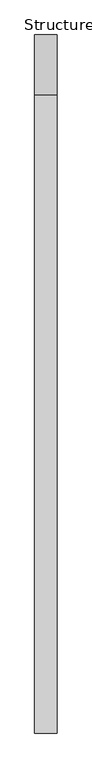
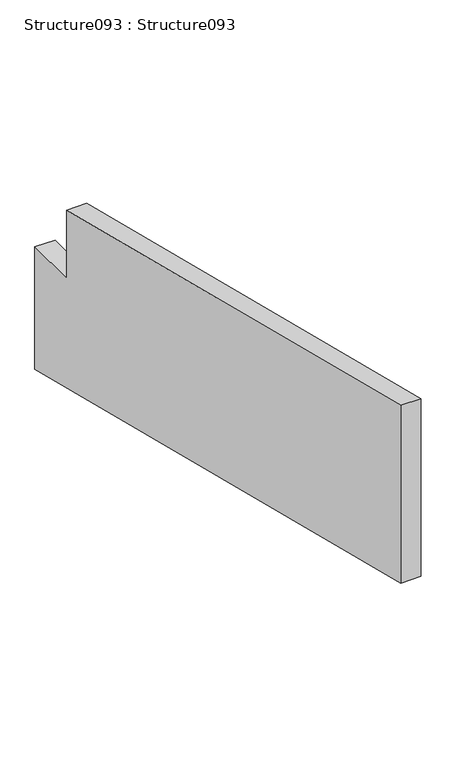
"""IFC4 building model written with IfcOpenShell, lengths in millimetres: proxy geometry, Structure093 : Structure093."""

from ifc_helpers import new_model, si_unit, frame, origin, place, context, project, spatial, polyline, outline, extrude, source, transform, mapped, element, save


def structure093_structure093_7474dfec(model_context):
    return source(origin(), model_context, "Body", "SweptSolid", [
        extrude(outline(polyline([(3064.1094171, 41796.3564587), (4341.2980909, 41477.0623881), (4341.2980909, 41318.4021881), (4461.9480928, 41318.4021881), (4461.9480928, 41032.8236949), (3064.1094171, 41382.2833638), (3064.1094171, 41796.3564587)])), frame((601.4870229, 0.0, 0.0), z_axis=(1.0, 0.0, 0.0), x_axis=(0.0, 1.0, 0.0)), (0.0, 0.0, 1.0), 44.45),
    ])


if __name__ == "__main__":
    model = new_model("IFC4")
    model_context = context("Model", 3, world=origin())
    ifc_project = project(units=[si_unit("LENGTHUNIT", "METRE", prefix="MILLI")], contexts=[model_context])
    site = spatial("IfcSite", under=ifc_project)
    building = spatial("IfcBuilding", under=site)
    placement = place(None, origin())
    structure093_structure093_shape = structure093_structure093_7474dfec(model_context)
    element("IfcBuildingElementProxy", 1, Name="Structure093 : Structure093", ObjectType="Structure093 : Structure093", at=placement, inside=building, context=model_context, shape_type="MappedRepresentation", body=[
        mapped(structure093_structure093_shape, transform((0.0, 0.0, 0.0), x_axis=(1.0, 0.0, 0.0), y_axis=(0.0, 1.0, 0.0), z_axis=(0.0, 0.0, 1.0))),
    ])
    save(model, "model.ifc")

# Revit data of these elements
# Type "Structure093 : Structure093"
#   NameOverride = "Structure093"
# Element 1 (IfcBuildingElementProxy, "Structure093 : Structure093")
#   Materials on its faces: "STRUCTURAL MEMBER (SEE DWGS)"
# Materials
#   "STRUCTURAL MEMBER (SEE DWGS)": class "Unassigned", colour RGB 214 178 158, transparency 0, Cost = 0
